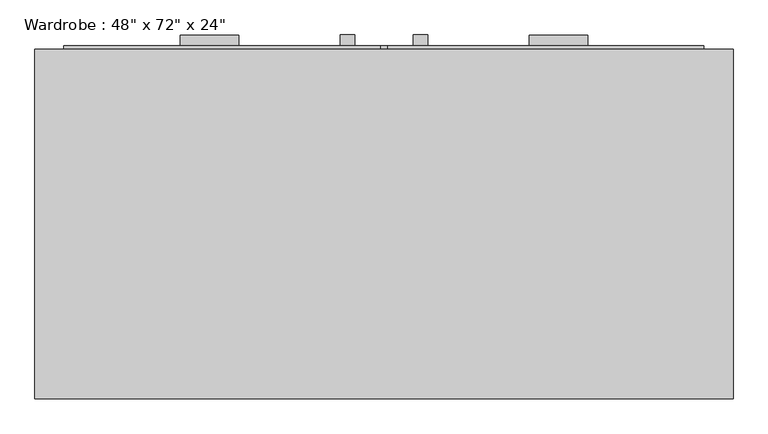
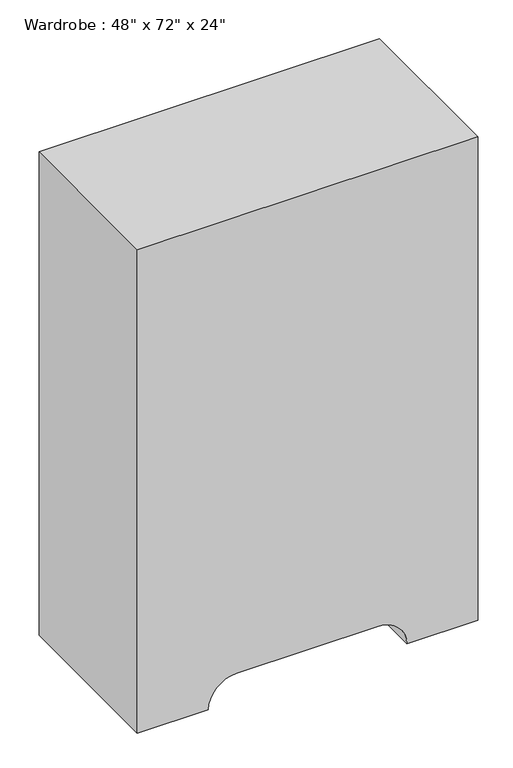
"""IFC4 building model written with IfcOpenShell, lengths in millimetres: furniture geometry."""

from ifc_helpers import new_model, si_unit, point, frame, frame_2d, origin, place, context, project, spatial, polyline, circle_curve, trimmed, segment, composite_curve, outline, extrude, source, transform, mapped, element, save


def furniture_49bbed1d(model_context):
    return source(origin(), model_context, "Body", "SweptSolid", [
        extrude(outline(composite_curve([segment(polyline([(0.0, 340.4067402), (1828.8, 340.4067402), (1828.8, -878.7932598), (0.0, -878.7932598), (0.0, -624.7932598)]), True, "CONTINUOUS"), segment(trimmed(circle_curve(frame_2d((0.0, -523.1932598)), 101.6), [point((0.0, -624.7932598))], [point((101.6, -523.1932598))], True, "CARTESIAN"), True, "CONTINUOUS"), segment(polyline([(101.6, -523.1932598), (101.6, -15.1932598)]), True, "CONTINUOUS"), segment(trimmed(circle_curve(frame_2d((0.0, -15.1932598)), 101.6), [point((101.6, -15.1932598))], [point((0.0, 86.4067402))], True, "CARTESIAN"), True, "CONTINUOUS"), segment(polyline([(0.0, 86.4067402), (0.0, 340.4067402)]), True, "CONTINUOUS")], self_intersect=False)), frame((0.0, 278.9388096, 0.0), z_axis=(0.0, 1.0, 0.0), x_axis=(0.0, 0.0, 1.0)), (0.0, 0.0, 1.0), 609.6),
        extrude(outline(polyline([(-319.9932598, 913.9388096), (-319.9932598, 894.8888096), (-345.3932598, 894.8888096), (-345.3932598, 913.9388096), (-319.9932598, 913.9388096)])), frame((0.0, 0.0, 1010.5571429), z_axis=(0.0, 0.0, 1.0), x_axis=(1.0, 0.0, 0.0)), (0.0, 0.0, 1.0), 101.6),
        extrude(outline(polyline([(-192.9932598, 913.9388096), (-192.9932598, 894.8888096), (-218.3932598, 894.8888096), (-218.3932598, 913.9388096), (-192.9932598, 913.9388096)])), frame((0.0, 0.0, 1010.5571429), z_axis=(0.0, 0.0, 1.0), x_axis=(1.0, 0.0, 0.0)), (0.0, 0.0, 1.0), 101.6),
        extrude(outline(polyline([(-523.1932598, 913.9388096), (-523.1932598, 894.8888096), (-624.7932598, 894.8888096), (-624.7932598, 913.9388096), (-523.1932598, 913.9388096)])), frame((0.0, 0.0, 534.3071429), z_axis=(0.0, 0.0, 1.0), x_axis=(1.0, 0.0, 0.0)), (0.0, 0.0, 1.0), 38.1),
        extrude(outline(polyline([(86.4067402, 913.9388096), (86.4067402, 894.8888096), (-15.1932598, 894.8888096), (-15.1932598, 913.9388096), (86.4067402, 913.9388096)])), frame((0.0, 0.0, 534.3071429), z_axis=(0.0, 0.0, 1.0), x_axis=(1.0, 0.0, 0.0)), (0.0, 0.0, 1.0), 38.1),
        extrude(outline(polyline([(86.4067402, 913.9388096), (86.4067402, 894.8888096), (-15.1932598, 894.8888096), (-15.1932598, 913.9388096), (86.4067402, 913.9388096)])), frame((0.0, 0.0, 302.0785714), z_axis=(0.0, 0.0, 1.0), x_axis=(1.0, 0.0, 0.0)), (0.0, 0.0, 1.0), 38.1),
        extrude(outline(polyline([(-523.1932598, 913.9388096), (-523.1932598, 894.8888096), (-624.7932598, 894.8888096), (-624.7932598, 913.9388096), (-523.1932598, 913.9388096)])), frame((0.0, 0.0, 302.0785714), z_axis=(0.0, 0.0, 1.0), x_axis=(1.0, 0.0, 0.0)), (0.0, 0.0, 1.0), 38.1),
        extrude(outline(polyline([(289.6067402, 894.8888096), (289.6067402, 888.5388096), (-827.9932598, 888.5388096), (-827.9932598, 894.8888096), (289.6067402, 894.8888096)])), frame((0.0, 0.0, 384.6285714), z_axis=(0.0, 0.0, 1.0), x_axis=(1.0, 0.0, 0.0)), (0.0, 0.0, 1.0), 213.1785714),
        extrude(outline(polyline([(289.6067402, 894.8888096), (289.6067402, 888.5388096), (-827.9932598, 888.5388096), (-827.9932598, 894.8888096), (289.6067402, 894.8888096)])), frame((0.0, 0.0, 152.4), z_axis=(0.0, 0.0, 1.0), x_axis=(1.0, 0.0, 0.0)), (0.0, 0.0, 1.0), 213.1785714),
        extrude(outline(polyline([(-275.5432598, 894.8888096), (-275.5432598, 888.5388096), (-827.9932598, 888.5388096), (-827.9932598, 894.8888096), (-275.5432598, 894.8888096)])), frame((0.0, 0.0, 616.8571429), z_axis=(0.0, 0.0, 1.0), x_axis=(1.0, 0.0, 0.0)), (0.0, 0.0, 1.0), 1161.1428571),
        extrude(outline(polyline([(289.6067402, 894.8888096), (289.6067402, 888.5388096), (-262.8432598, 888.5388096), (-262.8432598, 894.8888096), (289.6067402, 894.8888096)])), frame((0.0, 0.0, 616.8571429), z_axis=(0.0, 0.0, 1.0), x_axis=(1.0, 0.0, 0.0)), (0.0, 0.0, 1.0), 1161.1428571),
    ])


if __name__ == "__main__":
    model = new_model("IFC4")
    model_context = context("Model", 3, world=origin())
    ifc_project = project(units=[si_unit("LENGTHUNIT", "METRE", prefix="MILLI")], contexts=[model_context])
    site = spatial("IfcSite", under=ifc_project)
    building = spatial("IfcBuilding", under=site)
    placement = place(None, origin())
    furniture_shape = furniture_49bbed1d(model_context)
    element("IfcFurniture", 1, ObjectType="Wardrobe : 48\" x 72\" x 24\"", at=placement, inside=building, context=model_context, shape_type="MappedRepresentation", body=[
        mapped(furniture_shape, transform((0.0, 0.0, 0.0), x_axis=(1.0, 0.0, 0.0), y_axis=(0.0, 1.0, 0.0), z_axis=(0.0, 0.0, 1.0))),
    ])
    save(model, "model.ifc")

# Revit data of these elements
# Type "Wardrobe : 48\" x 72\" x 24\""
#   Model = "Entertainment Center"
#   Manufacturer = "Acme Funriture"
#   Assembly Code = "E2020200"
#   Depth = 2' - 0"
#   Height = 6' - 0"
#   Width = 4' - 0"
#   Material = Birch
#   Default Elevation = 0
# Element 1 (IfcFurniture, "Wardrobe : 48\" x 72\" x 24\"")
#   Materials on its faces: "Birch"
# Materials
#   "Birch": class "Wood", colour RGB 172 132 95, transparency 0, Description = "Betula Alleghaniensis", Cost = 0
